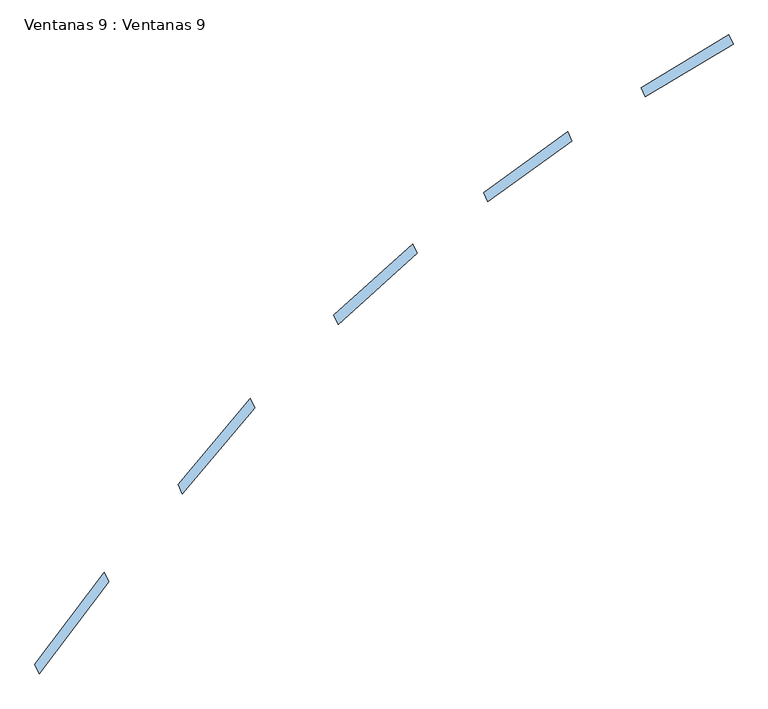
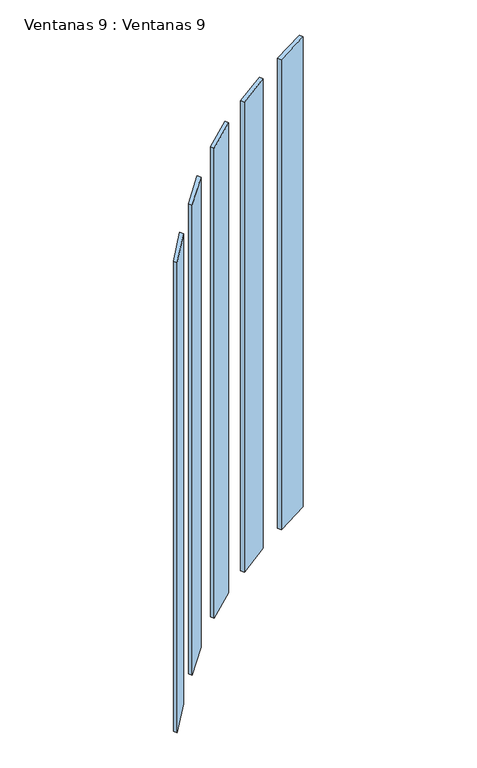
"""IFC4 building model written with IfcOpenShell, lengths in millimetres: window geometry, Ventanas 9 : Ventanas 9."""

from ifc_helpers import new_model, si_unit, frame, origin, place, context, project, spatial, polyline, outline, extrude, source, transform, mapped, element, save


def ventanas_9_ventanas_9_8d4206bf(model_context):
    return source(origin(), model_context, "Body", "SweptSolid", [
        extrude(outline(polyline([(353.6587096, 6581.2853175), (526.0364731, 6684.8603273), (534.4888384, 6666.7341715), (362.1110748, 6563.1591618), (353.6587096, 6581.2853175)])), frame((0.0, 0.0, 5975.0), z_axis=(0.0, 0.0, 1.0), x_axis=(1.0, 0.0, 0.0)), (0.0, 0.0, 1.0), 2556.7456382),
        extrude(outline(polyline([(44.5254237, 6374.8229217), (209.3572474, 6494.5802516), (217.8096126, 6476.4540959), (52.9777889, 6356.696766), (44.5254237, 6374.8229217)])), frame((0.0, 0.0, 5975.0), z_axis=(0.0, 0.0, 1.0), x_axis=(1.0, 0.0, 0.0)), (0.0, 0.0, 1.0), 2556.7456382),
        extrude(outline(polyline([(-249.7262128, 6134.0150225), (-94.3061292, 6273.9558943), (-85.853764, 6255.8297386), (-241.2738475, 6115.8888668), (-249.7262128, 6134.0150225)])), frame((0.0, 0.0, 5975.0), z_axis=(0.0, 0.0, 1.0), x_axis=(1.0, 0.0, 0.0)), (0.0, 0.0, 1.0), 2556.7456382),
        extrude(outline(polyline([(-555.4738246, 5801.0676371), (-413.6262935, 5970.1149418), (-405.1739283, 5951.988786), (-547.0214593, 5782.9414813), (-555.4738246, 5801.0676371)])), frame((0.0, 0.0, 5975.0), z_axis=(0.0, 0.0, 1.0), x_axis=(1.0, 0.0, 0.0)), (0.0, 0.0, 1.0), 2556.7456382),
        extrude(outline(polyline([(-836.8462456, 5447.2982061), (-700.5267113, 5628.2003382), (-692.0743461, 5610.0741824), (-828.3938804, 5429.1720504), (-836.8462456, 5447.2982061)])), frame((0.0, 0.0, 5975.0), z_axis=(0.0, 0.0, 1.0), x_axis=(1.0, 0.0, 0.0)), (0.0, 0.0, 1.0), 2556.7456382),
    ])


if __name__ == "__main__":
    model = new_model("IFC4")
    model_context = context("Model", 3, world=origin())
    ifc_project = project(units=[si_unit("LENGTHUNIT", "METRE", prefix="MILLI")], contexts=[model_context])
    site = spatial("IfcSite", under=ifc_project)
    building = spatial("IfcBuilding", under=site)
    placement = place(None, origin())
    ventanas_9_ventanas_9_shape = ventanas_9_ventanas_9_8d4206bf(model_context)
    element("IfcWindow", 1, ObjectType="Ventanas 9 : Ventanas 9", at=placement, inside=building, context=model_context, shape_type="MappedRepresentation", body=[
        mapped(ventanas_9_ventanas_9_shape, transform((0.0, 0.0, 0.0), x_axis=(1.0, 0.0, 0.0), y_axis=(0.0, 1.0, 0.0), z_axis=(0.0, 0.0, 1.0))),
    ])
    save(model, "model.ifc")

# Revit data of these elements
# Type "Ventanas 9 : Ventanas 9"
#   Type Mark = "50"
# Element 1 (IfcWindow, "Ventanas 9 : Ventanas 9")
#   Materials on its faces: "VIDRIO"
# Materials
#   "VIDRIO": class "Genérico", colour RGB 120 120 120, transparency 0, Cost = 0
